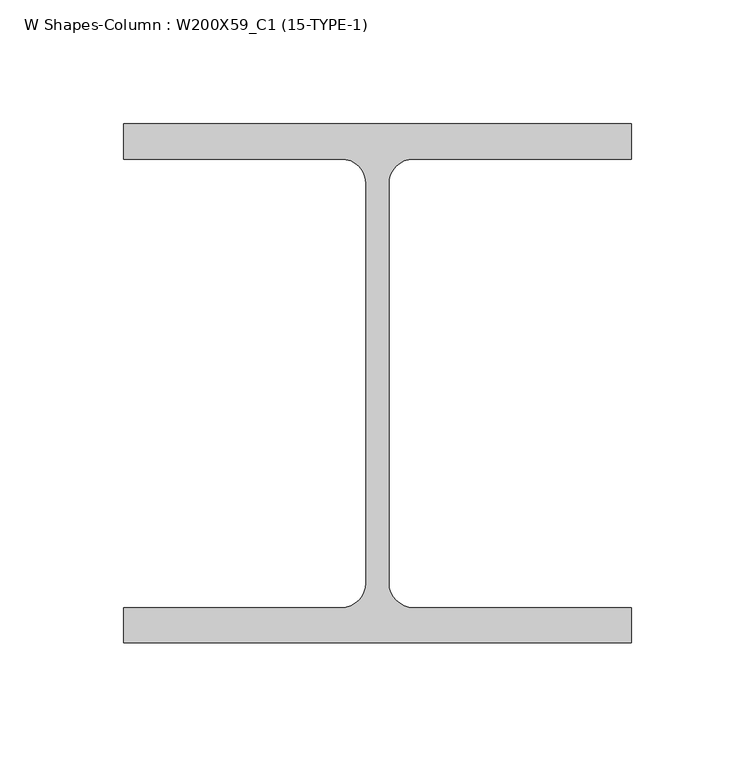
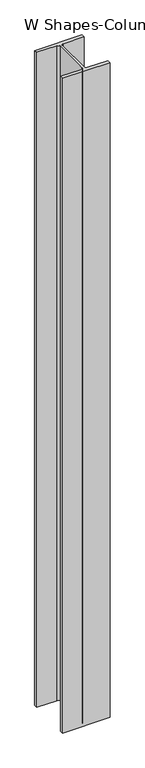
"""IFC4 building model written with IfcOpenShell, lengths in millimetres: column geometry, W Shapes-Column : W200X59_C1 (15-TYPE-1)."""

import ifcopenshell
import ifcopenshell.guid

model = None  # the IFC model being written
_history = None  # IfcOwnerHistory: only IFC2X3 demands one
_inside = {}  # id of a spatial element -> (the spatial element, [elements in it])
_under = {}  # id of a project, library or spatial element -> (it, [spatial elements below it])
_declared = {}  # id of a project -> (the project, [libraries it declares])
_typed = {}  # id of a type object -> (the type object, [elements of that type])
_made_of = {}  # id of a material, layer set ... -> (it, [elements and type objects made of it])


def new_model(schema):
    """Start an empty IFC model of exactly this schema.

    Asked for "IFC4X3", IfcOpenShell would pick the latest addendum, in which some entities
    have other attributes; the version numbers below select the first issue.
    IFC2X3 requires an IfcOwnerHistory on every rooted entity: one is made here for all.
    """
    global model, _history
    if schema == "IFC4X3":
        model = ifcopenshell.file(schema_version=(4, 3, 0, 0))
    else:
        model = ifcopenshell.file(schema=schema)
    _inside.clear()
    _under.clear()
    _declared.clear()
    _typed.clear()
    _made_of.clear()
    _history = None
    if model.schema == "IFC2X3":
        org = make("IfcOrganization", Name="unknown")
        user = make(
            "IfcPersonAndOrganization",
            ThePerson=make("IfcPerson", FamilyName="unknown"),
            TheOrganization=org,
        )
        app = make(
            "IfcApplication",
            ApplicationDeveloper=org,
            Version="unknown",
            ApplicationFullName="unknown",
            ApplicationIdentifier="unknown",
        )
        _history = make(
            "IfcOwnerHistory",
            OwningUser=user,
            OwningApplication=app,
            ChangeAction="ADDED",
            CreationDate=0,
        )
    return model


def make(cls, **values):
    """One entity of the class cls with the attributes given. An attribute that is None is left unset."""
    return model.create_entity(
        cls, **{name: value for name, value in values.items() if value is not None}
    )


def rooted(cls, **values):
    """An entity with a GlobalId (a new one), such as an element, a storey or a relation."""
    return make(cls, GlobalId=ifcopenshell.guid.new(), OwnerHistory=_history, **values)


def si_unit(unit_type, name, prefix=None):
    """IfcSIUnit, for example si_unit("LENGTHUNIT", "METRE", prefix="MILLI")."""
    return make("IfcSIUnit", UnitType=unit_type, Prefix=prefix, Name=name)


def assignment(units):
    """IfcUnitAssignment: the units of a project."""
    return None if units is None else make("IfcUnitAssignment", Units=units)


def point(xyz):
    """IfcCartesianPoint."""
    return None if xyz is None else make("IfcCartesianPoint", Coordinates=xyz)


def direction(xyz):
    """IfcDirection."""
    return None if xyz is None else make("IfcDirection", DirectionRatios=xyz)


def frame(location, z_axis=None, x_axis=None):
    """IfcAxis2Placement3D, a coordinate frame: its origin and axes. An axis left out is left unset."""
    return make(
        "IfcAxis2Placement3D",
        Location=point(location),
        Axis=direction(z_axis),
        RefDirection=direction(x_axis),
    )


def frame_2d(location, x_axis=None):
    """IfcAxis2Placement2D, a coordinate frame in the plane: its origin and x axis."""
    return make(
        "IfcAxis2Placement2D", Location=point(location), RefDirection=direction(x_axis)
    )


def origin():
    """The frame at (0, 0, 0) with its axes left unset."""
    return frame((0.0, 0.0, 0.0))


def place(relative_to, where):
    """IfcLocalPlacement: puts the frame where relative to a parent placement (None: the world)."""
    return make(
        "IfcLocalPlacement", PlacementRelTo=relative_to, RelativePlacement=where
    )


def context(
    kind, dimensions, precision=None, world=None, true_north=None, identifier=None
):
    """IfcGeometricRepresentationContext, for example the 3D "Model" context."""
    return make(
        "IfcGeometricRepresentationContext",
        ContextIdentifier=identifier,
        ContextType=kind,
        CoordinateSpaceDimension=dimensions,
        Precision=precision,
        WorldCoordinateSystem=world,
        TrueNorth=true_north,
    )


def project(units=None, contexts=None):
    """IfcProject with its units and contexts."""
    return rooted(
        "IfcProject",
        Name="project",
        RepresentationContexts=contexts,
        UnitsInContext=assignment(units),
    )


def spatial(cls, under=None, at=None, **own):
    """A site, building, storey or space (cls), placed at a placement, below another one or the project."""
    s = rooted(cls, ObjectPlacement=at, **own)
    if under is not None:
        _under.setdefault(under.id(), (under, []))[1].append(s)
    return s


def polyline(points):
    """IfcPolyline through the points."""
    return make("IfcPolyline", Points=[point(p) for p in points])


def circle_curve(where, radius):
    """IfcCircle in the frame where."""
    return make("IfcCircle", Position=where, Radius=radius)


def trimmed(basis, trim1, trim2, sense, master):
    """IfcTrimmedCurve: the piece of a basis curve between two trims."""
    return make(
        "IfcTrimmedCurve",
        BasisCurve=basis,
        Trim1=trim1,
        Trim2=trim2,
        SenseAgreement=sense,
        MasterRepresentation=master,
    )


def segment(curve, same_sense, transition):
    """IfcCompositeCurveSegment."""
    return make(
        "IfcCompositeCurveSegment",
        Transition=transition,
        SameSense=same_sense,
        ParentCurve=curve,
    )


def composite_curve(segments, self_intersect=None):
    """IfcCompositeCurve: segments joined end to end."""
    return make("IfcCompositeCurve", Segments=segments, SelfIntersect=self_intersect)


def outline(outer, holes=None, kind="AREA"):
    """IfcArbitraryClosedProfileDef: a profile drawn as a closed curve; with holes, ...WithVoids."""
    if holes is None:
        return make("IfcArbitraryClosedProfileDef", ProfileType=kind, OuterCurve=outer)
    return make(
        "IfcArbitraryProfileDefWithVoids",
        ProfileType=kind,
        OuterCurve=outer,
        InnerCurves=holes,
    )


def extrude(swept, where, along, depth):
    """IfcExtrudedAreaSolid: the profile swept, set in the frame where, extruded along a direction by depth."""
    return make(
        "IfcExtrudedAreaSolid",
        SweptArea=swept,
        Position=where,
        ExtrudedDirection=direction(along),
        Depth=depth,
    )


def shape(context_of_items, identifier, shape_type, items):
    """IfcShapeRepresentation: the items that make up one representation, for example the "Body"."""
    return make(
        "IfcShapeRepresentation",
        ContextOfItems=context_of_items,
        RepresentationIdentifier=identifier,
        RepresentationType=shape_type,
        Items=items,
    )


def source(mapping_origin, context_of_items, identifier, shape_type, items):
    """IfcRepresentationMap: a shape defined once, which mapped items show again and again."""
    return make(
        "IfcRepresentationMap",
        MappingOrigin=mapping_origin,
        MappedRepresentation=shape(context_of_items, identifier, shape_type, items),
    )


def transform(
    local_origin,
    x_axis=None,
    y_axis=None,
    z_axis=None,
    scale=None,
    scale2=None,
    scale3=None,
    uniform=True,
):
    """IfcCartesianTransformationOperator3D, or its non-uniform kind. x_axis, y_axis, z_axis: its Axis1, 2, 3."""
    if uniform:
        return make(
            "IfcCartesianTransformationOperator3D",
            Axis1=direction(x_axis),
            Axis2=direction(y_axis),
            LocalOrigin=point(local_origin),
            Scale=scale,
            Axis3=direction(z_axis),
        )
    return make(
        "IfcCartesianTransformationOperator3DnonUniform",
        Axis1=direction(x_axis),
        Axis2=direction(y_axis),
        LocalOrigin=point(local_origin),
        Scale=scale,
        Axis3=direction(z_axis),
        Scale2=scale2,
        Scale3=scale3,
    )


def mapped(mapping_source, mapping_target):
    """IfcMappedItem: shows the shape of a source again, moved by a transform."""
    return make(
        "IfcMappedItem", MappingSource=mapping_source, MappingTarget=mapping_target
    )


def made_of(thing, what):
    """Note that an element or type object is made of a material, layer set ...; save() writes the relation."""
    if what is not None:
        _made_of.setdefault(what.id(), (what, []))[1].append(thing)
    return thing


def element(
    cls,
    number,
    at=None,
    inside=None,
    cuts=None,
    type_object=None,
    material=None,
    context=None,
    identifier="Body",
    shape_type=None,
    held_by="IfcProductDefinitionShape",
    body=None,
    shapes=None,
    **own,
):
    """One element of the class cls, such as IfcWall. Its Tag is "e" and its number.

    at: its placement. inside: the storey or other place that contains it. cuts: it is an
    opening in that element (IfcRelVoidsElement). A single representation is given by context,
    identifier, shape_type and body (its items); several are given by shapes. held_by: the class
    of the entity that holds the representations. save() writes the other relations.
    """
    e = rooted(cls, Tag="e%d" % number, ObjectPlacement=at, **own)
    if body is not None:
        shapes = [shape(context, identifier, shape_type, body)]
    if shapes is not None:
        e.Representation = make(held_by, Representations=shapes)
    if inside is not None:
        _inside.setdefault(inside.id(), (inside, []))[1].append(e)
    if cuts is not None:
        rooted(
            "IfcRelVoidsElement", RelatingBuildingElement=cuts, RelatedOpeningElement=e
        )
    if type_object is not None:
        _typed.setdefault(type_object.id(), (type_object, []))[1].append(e)
    return made_of(e, material)


def aggregate(whole, parts):
    """IfcRelAggregates: a whole, such as a stair, and the parts it consists of."""
    return rooted("IfcRelAggregates", RelatingObject=whole, RelatedObjects=parts)


def save(model, path):
    """Write the relations noted so far, then the file.

    IfcRelAggregates (storeys below a building ...), IfcRelContainedInSpatialStructure (elements
    in a storey), IfcRelDefinesByType, IfcRelAssociatesMaterial and IfcRelDeclares: one each for
    every whole, place, type object, material and project.
    """
    for whole, parts in _under.values():
        aggregate(whole, parts)
    for where, things in _inside.values():
        rooted(
            "IfcRelContainedInSpatialStructure",
            RelatedElements=things,
            RelatingStructure=where,
        )
    for kind, things in _typed.values():
        rooted("IfcRelDefinesByType", RelatedObjects=things, RelatingType=kind)
    for what, things in _made_of.values():
        rooted("IfcRelAssociatesMaterial", RelatedObjects=things, RelatingMaterial=what)
    for by, libraries in _declared.values():
        rooted("IfcRelDeclares", RelatingContext=by, RelatedDefinitions=libraries)
    model.write(path)


def w_shapes_column_w200x59_c1_15_type_1_67f7008f(model_context):
    return source(origin(), model_context, "Body", "SweptSolid", [
        extrude(outline(composite_curve([segment(polyline([(102.489, 104.775), (102.489, 90.551), (14.5796, 90.551)]), True, "CONTINUOUS"), segment(trimmed(circle_curve(frame_2d((14.5796, 80.5434)), 10.0076), [point((14.5796, 90.551))], [point((4.572, 80.5434))], True, "CARTESIAN"), True, "CONTINUOUS"), segment(polyline([(4.572, 80.5434), (4.572, -80.5434)]), True, "CONTINUOUS"), segment(trimmed(circle_curve(frame_2d((14.5796, -80.5434)), 10.0076), [point((4.572, -80.5434))], [point((14.5796, -90.551))], True, "CARTESIAN"), True, "CONTINUOUS"), segment(polyline([(14.5796, -90.551), (102.489, -90.551), (102.489, -104.775), (-102.489, -104.775), (-102.489, -90.551), (-14.5796, -90.551)]), True, "CONTINUOUS"), segment(trimmed(circle_curve(frame_2d((-14.5796, -80.5434)), 10.0076), [point((-14.5796, -90.551))], [point((-4.572, -80.5434))], True, "CARTESIAN"), True, "CONTINUOUS"), segment(polyline([(-4.572, -80.5434), (-4.572, 80.5434)]), True, "CONTINUOUS"), segment(trimmed(circle_curve(frame_2d((-14.5796, 80.5434)), 10.0076), [point((-4.572, 80.5434))], [point((-14.5796, 90.551))], True, "CARTESIAN"), True, "CONTINUOUS"), segment(polyline([(-14.5796, 90.551), (-102.489, 90.551), (-102.489, 104.775), (102.489, 104.775)]), True, "CONTINUOUS")], self_intersect=False)), frame((0.0, 0.0, 3220.0), z_axis=(0.0, 0.0, 1.0), x_axis=(1.0, 0.0, 0.0)), (0.0, 0.0, 1.0), 3000.0),
    ])


if __name__ == "__main__":
    model = new_model("IFC4")
    model_context = context("Model", 3, world=origin())
    ifc_project = project(units=[si_unit("LENGTHUNIT", "METRE", prefix="MILLI")], contexts=[model_context])
    site = spatial("IfcSite", under=ifc_project)
    building = spatial("IfcBuilding", under=site)
    placement = place(None, origin())
    w_shapes_column_w200x59_c1_15_type_1_shape = w_shapes_column_w200x59_c1_15_type_1_67f7008f(model_context)
    element("IfcColumn", 1, ObjectType="W Shapes-Column : W200X59_C1 (15-TYPE-1)", at=placement, inside=building, context=model_context, shape_type="MappedRepresentation", body=[
        mapped(w_shapes_column_w200x59_c1_15_type_1_shape, transform((0.0, 0.0, 0.0), x_axis=(1.0, 0.0, 0.0), y_axis=(0.0, 1.0, 0.0), z_axis=(0.0, 0.0, 1.0))),
    ])
    save(model, "model.ifc")

# Revit data of these elements
# Type "W Shapes-Column : W200X59_C1 (15-TYPE-1)"
#   Section Name Key = "W8x40"
#   Assembly Code = "B10"
#   Width = 20.4978 cm
#   Web Thickness = 0.9144 cm
#   Web Fillet = 1.0008 cm
#   Warping Constant = 194957.0 cm⁶
#   Torsional Moment of Inertia = 46.6179 cm⁴
#   Section Area = 75.4837 cm²
#   Plastic Modulus weak axis = 303.161 cm³
#   Plastic Modulus strong axis = 652.205 cm³
#   Perimeter = 1.20396 m²/m
#   Nominal Weight = 59.5266 kgf/m
#   Moment of Inertia weak axis = 2043.70 cm⁴
#   Moment of Inertia strong axis = 6076.98 cm⁴
#   Height = 20.955 cm
#   Flange Thickness = 1.4224 cm
#   Elastic Modulus weak axis = 199.922 cm³
#   Elastic Modulus strong axis = 581.741 cm³
#   Clear Web Height = 19.05 cm
#   Centroid Vertical = 10.4775 cm
#   Centroid Horizontal = 10.2489 cm
#   Bolt Spacing = 13.97 cm
#   Structural Material [instance default] = Steel ASTM A992
#   Principal Axes Angle = 0
# Element 1 (IfcColumn, "W Shapes-Column : W200X59_C1 (15-TYPE-1)")
#   Structural Material = none
# Materials
#   "Steel ASTM A992": class "Metal", colour RGB 199 199 199, transparency 0, Description = "Structural steel 50ksi", Cost = 0
